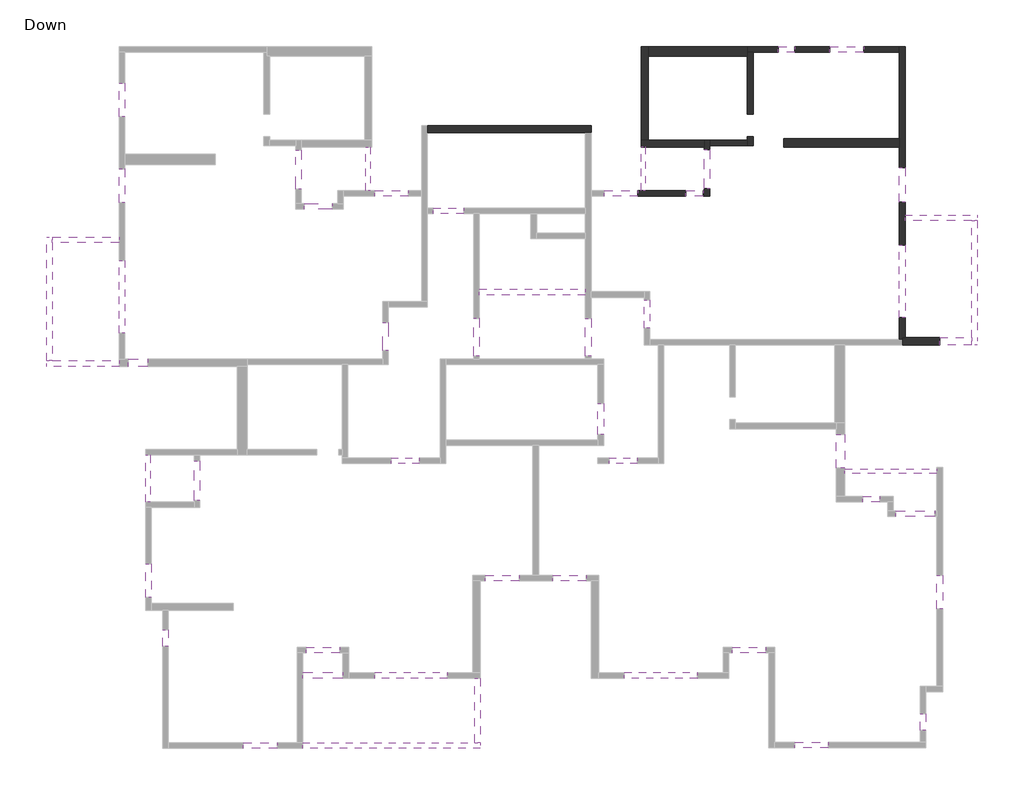
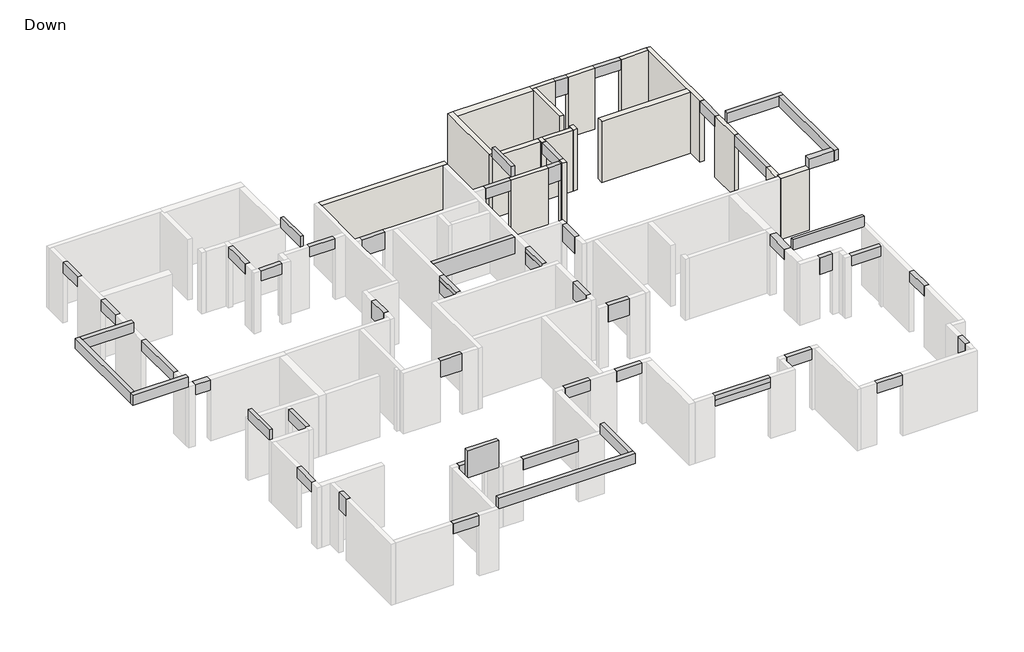
# One storey, part 3 of 3: 52 beams, 19 walls.
"""IFC4 building model written with IfcOpenShell, lengths in millimetres."""

from ifc_helpers import new_model, si_unit, frame, origin, place, context, project, spatial, polyline, outline, extrude, faceted_brep, element, save

model = new_model("IFC4")

# Units and contexts
model_context = context("Model", 3, world=origin())
ifc_project = project(units=[si_unit("LENGTHUNIT", "METRE", prefix="MILLI")], contexts=[model_context])

# Site, building, storey
site = spatial("IfcSite", under=ifc_project)
building = spatial("IfcBuilding", under=site)
storey = spatial("IfcBuildingStorey", under=building, Name="Down", Elevation=0.0)

# Beams
placement = place(None, origin())
element("IfcBeam", 1, ObjectType="Concrete Rectengular Beam : 15/50", at=placement, inside=storey, context=model_context, shape_type="SweptSolid", body=[
    extrude(outline(polyline([(18937.905294, -3693.5538503), (18937.905294, -3843.5538503), (15639.9526685, -3843.5538503), (15639.9526685, -3693.5538503), (18937.905294, -3693.5538503)])), frame((0.0, 0.0, 3000.0), z_axis=(0.0, 0.0, 1.0), x_axis=(1.0, 0.0, 0.0)), (0.0, 0.0, 1.0), 500.0),
])
element("IfcBeam", 2, ObjectType="Concrete Rectengular Beam : 15/50", at=placement, inside=storey, context=model_context, shape_type="SweptSolid", body=[
    extrude(outline(polyline([(8357.905294, 7842.0164502), (8507.905294, 7842.0164502), (8507.905294, 6284.3445962), (8357.905294, 6284.3445962), (8357.905294, 7842.0164502)])), frame((0.0, 0.0, 3000.0), z_axis=(0.0, 0.0, 1.0), x_axis=(1.0, 0.0, 0.0)), (0.0, 0.0, 1.0), 500.0),
])
element("IfcBeam", 3, ObjectType="Concrete Rectengular Beam : 15/50", at=placement, inside=storey, context=model_context, shape_type="SweptSolid", body=[
    extrude(outline(polyline([(-1489.8370837, 7836.068874), (-1339.8370837, 7836.068874), (-1339.8370837, 6280.1520062), (-1489.8370837, 6280.1520062), (-1489.8370837, 7836.068874)])), frame((0.0, 0.0, 3000.0), z_axis=(0.0, 0.0, 1.0), x_axis=(1.0, 0.0, 0.0)), (0.0, 0.0, 1.0), 500.0),
])
element("IfcBeam", 4, ObjectType="Concrete Rectengular Beam : 15/50", at=placement, inside=storey, context=model_context, shape_type="SweptSolid", body=[
    extrude(outline(polyline([(-9364.7328942, -3194.7427075), (-9214.7328942, -3194.7427075), (-9214.7328942, -4872.9835498), (-9364.7328942, -4872.9835498), (-9364.7328942, -3194.7427075)])), frame((0.0, 0.0, 3000.0), z_axis=(0.0, 0.0, 1.0), x_axis=(1.0, 0.0, 0.0)), (0.0, 0.0, 1.0), 500.0),
])
element("IfcBeam", 5, ObjectType="Concrete Rectengular Beam : 20/133", at=placement, inside=storey, context=model_context, shape_type="SweptSolid", body=[
    extrude(outline(polyline([(-3754.594706, -11177.9835498), (-3754.594706, -10977.9835498), (-2314.594706, -10977.9835498), (-2314.594706, -11177.9835498), (-3754.594706, -11177.9835498)])), frame((0.0, 0.0, 3000.0), z_axis=(0.0, 0.0, 1.0), x_axis=(1.0, 0.0, 0.0)), (0.0, 0.0, 1.0), 1330.0),
])
element("IfcBeam", 6, ObjectType="Concrete Rectengular Beam : 20/50", at=placement, inside=storey, context=model_context, shape_type="Brep", body=[
    faceted_brep([(-3999.8370837, 7726.5624033, 3000.0), (-3799.8370837, 7726.5624033, 3000.0), (-3799.8370837, 7726.5624033, 2500.0), (-3999.8370837, 7726.5624033, 2500.0), (-3999.8370837, 7215.1187953, 3000.0), (-3999.8370837, 6335.1520062, 3000.0), (-3799.8370837, 6335.1520062, 3000.0), (-3799.8370837, 6335.1520062, 2500.0), (-3999.8370837, 6335.1520062, 2500.0)], [[[0, 1, 2, 3]], [[1, 0, 4, 5, 6]], [[2, 1, 6, 7]], [[3, 2, 7, 8]], [[0, 3, 8, 5, 4]], [[6, 5, 8, 7]]]),
])
element("IfcBeam", 7, ObjectType="Concrete Rectengular Beam : 20/50", at=placement, inside=storey, context=model_context, shape_type="SweptSolid", body=[
    extrude(outline(polyline([(-2696.679593, 5815.1520062), (-2696.679593, 5615.1520062), (-3696.679593, 5615.1520062), (-3696.679593, 5815.1520062), (-2696.679593, 5815.1520062)])), frame((0.0, 0.0, 2500.0), z_axis=(0.0, 0.0, 1.0), x_axis=(1.0, 0.0, 0.0)), (0.0, 0.0, 1.0), 500.0),
])
element("IfcBeam", 8, ObjectType="Concrete Rectengular Beam : 20/50", at=placement, inside=storey, context=model_context, shape_type="SweptSolid", body=[
    extrude(outline(polyline([(28.320407, 6280.1520062), (28.320407, 6080.1520062), (-1171.679593, 6080.1520062), (-1171.679593, 6280.1520062), (28.320407, 6280.1520062)])), frame((0.0, 0.0, 2500.0), z_axis=(0.0, 0.0, 1.0), x_axis=(1.0, 0.0, 0.0)), (0.0, 0.0, 1.0), 500.0),
])
element("IfcBeam", 9, ObjectType="Concrete Rectengular Beam : 20/50", at=placement, inside=storey, context=model_context, shape_type="SweptSolid", body=[
    extrude(outline(polyline([(-10319.6462524, 10130.5632806), (-10119.6462524, 10130.5632806), (-10119.6462524, 8930.3987709), (-10319.6462524, 8930.3987709), (-10319.6462524, 10130.5632806)])), frame((0.0, 0.0, 2500.0), z_axis=(0.0, 0.0, 1.0), x_axis=(1.0, 0.0, 0.0)), (0.0, 0.0, 1.0), 500.0),
])
element("IfcBeam", 10, ObjectType="Concrete Rectengular Beam : 20/50", at=placement, inside=storey, context=model_context, shape_type="SweptSolid", body=[
    extrude(outline(polyline([(-10319.6462524, 7055.0094311), (-10119.6462524, 7055.0094311), (-10119.6462524, 5854.8449214), (-10319.6462524, 5854.8449214), (-10319.6462524, 7055.0094311)])), frame((0.0, 0.0, 2500.0), z_axis=(0.0, 0.0, 1.0), x_axis=(1.0, 0.0, 0.0)), (0.0, 0.0, 1.0), 500.0),
])
element("IfcBeam", 11, ObjectType="Concrete Rectengular Beam : 20/50", at=placement, inside=storey, context=model_context, shape_type="SweptSolid", body=[
    extrude(outline(polyline([(-10319.6462524, 3780.4865094), (-10119.6462524, 3780.4865094), (-10119.6462524, 1181.1884177), (-10319.6462524, 1181.1884177), (-10319.6462524, 3780.4865094)])), frame((0.0, 0.0, 2500.0), z_axis=(0.0, 0.0, 1.0), x_axis=(1.0, 0.0, 0.0)), (0.0, 0.0, 1.0), 500.0),
])
element("IfcBeam", 12, ObjectType="Concrete Rectengular Beam : 20/50", at=placement, inside=storey, context=model_context, shape_type="SweptSolid", body=[
    extrude(outline(polyline([(-7634.594706, -3392.9835498), (-7434.594706, -3392.9835498), (-7434.594706, -4812.9835498), (-7634.594706, -4812.9835498), (-7634.594706, -3392.9835498)])), frame((0.0, 0.0, 2500.0), z_axis=(0.0, 0.0, 1.0), x_axis=(1.0, 0.0, 0.0)), (0.0, 0.0, 1.0), 500.0),
])
element("IfcBeam", 13, ObjectType="Concrete Rectengular Beam : 20/50", at=placement, inside=storey, context=model_context, shape_type="SweptSolid", body=[
    extrude(outline(polyline([(-9364.594706, -7092.9835498), (-9164.594706, -7092.9835498), (-9164.594706, -8292.9835498), (-9364.594706, -8292.9835498), (-9364.594706, -7092.9835498)])), frame((0.0, 0.0, 2500.0), z_axis=(0.0, 0.0, 1.0), x_axis=(1.0, 0.0, 0.0)), (0.0, 0.0, 1.0), 500.0),
])
element("IfcBeam", 14, ObjectType="Concrete Rectengular Beam : 20/50", at=placement, inside=storey, context=model_context, shape_type="SweptSolid", body=[
    extrude(outline(polyline([(-5884.594706, -13682.9835498), (-5884.594706, -13482.9835498), (-4664.594706, -13482.9835498), (-4664.594706, -13682.9835498), (-5884.594706, -13682.9835498)])), frame((0.0, 0.0, 2500.0), z_axis=(0.0, 0.0, 1.0), x_axis=(1.0, 0.0, 0.0)), (0.0, 0.0, 1.0), 500.0),
])
element("IfcBeam", 15, ObjectType="Concrete Rectengular Beam : 20/50", at=placement, inside=storey, context=model_context, shape_type="SweptSolid", body=[
    extrude(outline(polyline([(-3634.594706, -10272.9835498), (-3634.594706, -10072.9835498), (-2434.594706, -10072.9835498), (-2434.594706, -10272.9835498), (-3634.594706, -10272.9835498)])), frame((0.0, 0.0, 2500.0), z_axis=(0.0, 0.0, 1.0), x_axis=(1.0, 0.0, 0.0)), (0.0, 0.0, 1.0), 500.0),
])
element("IfcBeam", 16, ObjectType="Concrete Rectengular Beam : 20/50", at=placement, inside=storey, context=model_context, shape_type="SweptSolid", body=[
    extrude(outline(polyline([(-1184.594706, -11177.9835498), (-1184.594706, -10977.9835498), (1415.405294, -10977.9835498), (1415.405294, -11177.9835498), (-1184.594706, -11177.9835498)])), frame((0.0, 0.0, 2500.0), z_axis=(0.0, 0.0, 1.0), x_axis=(1.0, 0.0, 0.0)), (0.0, 0.0, 1.0), 500.0),
])
element("IfcBeam", 17, ObjectType="Concrete Rectengular Beam : 20/50", at=placement, inside=storey, context=model_context, shape_type="SweptSolid", body=[
    extrude(outline(polyline([(2785.405294, -7702.9835498), (2785.405294, -7502.9835498), (3985.405294, -7502.9835498), (3985.405294, -7702.9835498), (2785.405294, -7702.9835498)])), frame((0.0, 0.0, 2500.0), z_axis=(0.0, 0.0, 1.0), x_axis=(1.0, 0.0, 0.0)), (0.0, 0.0, 1.0), 500.0),
])
element("IfcBeam", 18, ObjectType="Concrete Rectengular Beam : 20/50", at=placement, inside=storey, context=model_context, shape_type="SweptSolid", body=[
    extrude(outline(polyline([(5185.405294, -7702.9835498), (5185.405294, -7502.9835498), (6385.405294, -7502.9835498), (6385.405294, -7702.9835498), (5185.405294, -7702.9835498)])), frame((0.0, 0.0, 2500.0), z_axis=(0.0, 0.0, 1.0), x_axis=(1.0, 0.0, 0.0)), (0.0, 0.0, 1.0), 500.0),
])
element("IfcBeam", 19, ObjectType="Concrete Rectengular Beam : 20/50", at=placement, inside=storey, context=model_context, shape_type="SweptSolid", body=[
    extrude(outline(polyline([(8239.9948169, 6284.3445962), (8239.9948169, 6084.3445962), (7043.320407, 6084.3445962), (7043.320407, 6284.3445962), (8239.9948169, 6284.3445962)])), frame((0.0, 0.0, 2500.0), z_axis=(0.0, 0.0, 1.0), x_axis=(1.0, 0.0, 0.0)), (0.0, 0.0, 1.0), 500.0),
])
element("IfcBeam", 20, ObjectType="Concrete Rectengular Beam : 20/50", at=placement, inside=storey, context=model_context, shape_type="Brep", body=[
    faceted_brep([(10617.905294, 7752.0164502, 3000.0), (10817.905294, 7752.0164502, 3000.0), (10817.905294, 7752.0164502, 2780.0), (10817.905294, 7752.0164502, 2500.0), (10617.905294, 7752.0164502, 2500.0), (10617.905294, 6354.3445962, 3000.0), (10817.905294, 6354.3445962, 3000.0), (10817.905294, 6354.3445962, 2500.0), (10617.905294, 6354.3445962, 2500.0)], [[[0, 1, 2, 3, 4]], [[1, 0, 5, 6]], [[2, 1, 6, 7, 3]], [[4, 3, 7, 8]], [[0, 4, 8, 5]], [[6, 5, 8, 7]]]),
])
element("IfcBeam", 21, ObjectType="Concrete Rectengular Beam : 20/50", at=placement, inside=storey, context=model_context, shape_type="SweptSolid", body=[
    extrude(outline(polyline([(16317.905294, 11432.0164502), (16317.905294, 11232.0164502), (15097.905294, 11232.0164502), (15097.905294, 11432.0164502), (16317.905294, 11432.0164502)])), frame((0.0, 0.0, 2500.0), z_axis=(0.0, 0.0, 1.0), x_axis=(1.0, 0.0, 0.0)), (0.0, 0.0, 1.0), 500.0),
])
element("IfcBeam", 22, ObjectType="Concrete Rectengular Beam : 20/50", at=placement, inside=storey, context=model_context, shape_type="SweptSolid", body=[
    extrude(outline(polyline([(17797.905294, 5872.0164502), (17597.905294, 5872.0164502), (17597.905294, 7092.0164502), (17797.905294, 7092.0164502), (17797.905294, 5872.0164502)])), frame((0.0, 0.0, 2500.0), z_axis=(0.0, 0.0, 1.0), x_axis=(1.0, 0.0, 0.0)), (0.0, 0.0, 1.0), 500.0),
])
element("IfcBeam", 23, ObjectType="Concrete Rectengular Beam : 20/50", at=placement, inside=storey, context=model_context, shape_type="SweptSolid", body=[
    extrude(outline(polyline([(17797.905294, 1732.0164502), (17597.905294, 1732.0164502), (17597.905294, 4332.0164502), (17797.905294, 4332.0164502), (17797.905294, 1732.0164502)])), frame((0.0, 0.0, 2500.0), z_axis=(0.0, 0.0, 1.0), x_axis=(1.0, 0.0, 0.0)), (0.0, 0.0, 1.0), 500.0),
])
element("IfcBeam", 24, ObjectType="Concrete Rectengular Beam : 20/50", at=placement, inside=storey, context=model_context, shape_type="SweptSolid", body=[
    extrude(outline(polyline([(18857.905294, -5182.9835498), (18857.905294, -5382.9835498), (17457.905294, -5382.9835498), (17457.905294, -5182.9835498), (18857.905294, -5182.9835498)])), frame((0.0, 0.0, 2500.0), z_axis=(0.0, 0.0, 1.0), x_axis=(1.0, 0.0, 0.0)), (0.0, 0.0, 1.0), 500.0),
])
element("IfcBeam", 25, ObjectType="Concrete Rectengular Beam : 20/50", at=placement, inside=storey, context=model_context, shape_type="SweptSolid", body=[
    extrude(outline(polyline([(19137.905294, -8697.9835498), (18937.905294, -8697.9835498), (18937.905294, -7497.9835498), (19137.905294, -7497.9835498), (19137.905294, -8697.9835498)])), frame((0.0, 0.0, 2500.0), z_axis=(0.0, 0.0, 1.0), x_axis=(1.0, 0.0, 0.0)), (0.0, 0.0, 1.0), 500.0),
])
element("IfcBeam", 26, ObjectType="Concrete Rectengular Beam : 20/50", at=placement, inside=storey, context=model_context, shape_type="SweptSolid", body=[
    extrude(outline(polyline([(13857.905294, -13677.9835498), (13857.905294, -13477.9835498), (15057.905294, -13477.9835498), (15057.905294, -13677.9835498), (13857.905294, -13677.9835498)])), frame((0.0, 0.0, 2500.0), z_axis=(0.0, 0.0, 1.0), x_axis=(1.0, 0.0, 0.0)), (0.0, 0.0, 1.0), 500.0),
])
element("IfcBeam", 27, ObjectType="Concrete Rectengular Beam : 20/50", at=placement, inside=storey, context=model_context, shape_type="SweptSolid", body=[
    extrude(outline(polyline([(11607.905294, -10277.9835498), (11607.905294, -10077.9835498), (12807.905294, -10077.9835498), (12807.905294, -10277.9835498), (11607.905294, -10277.9835498)])), frame((0.0, 0.0, 2500.0), z_axis=(0.0, 0.0, 1.0), x_axis=(1.0, 0.0, 0.0)), (0.0, 0.0, 1.0), 500.0),
])
element("IfcBeam", 28, ObjectType="Concrete Rectengular Beam : 20/50", at=placement, inside=storey, context=model_context, shape_type="SweptSolid", body=[
    extrude(outline(polyline([(-11172.9835498, 3000.0), (-10977.9835498, 3000.0), (-10977.9835498, 2500.0), (-11177.9835498, 2500.0), (-11177.9835498, 2780.0), (-11172.9835498, 2780.0), (-11172.9835498, 3000.0)])), frame((7755.405294, 0.0, 0.0), z_axis=(1.0, 0.0, 0.0), x_axis=(0.0, 1.0, 0.0)), (0.0, 0.0, 1.0), 2602.5),
])
element("IfcBeam", 29, ObjectType="Concrete Rectengular Beam : 20/50", at=placement, inside=storey, context=model_context, shape_type="Brep", body=[
    faceted_brep([(-3754.594706, -13482.9835498, 3500.0), (-3754.594706, -13482.9835498, 3000.0), (-3754.594706, -13682.9835498, 3000.0), (-3754.594706, -13682.9835498, 3500.0), (2605.405294, -13682.9835498, 3500.0), (2605.405294, -13482.9835498, 3500.0), (2405.405294, -13482.9835498, 3500.0), (2605.405294, -13682.9835498, 3000.0), (2405.405294, -13482.9835498, 3000.0), (2605.405294, -13482.9835498, 3000.0)], [[[0, 1, 2, 3]], [[0, 3, 4, 5, 6]], [[3, 2, 7, 4]], [[2, 1, 8, 9, 7]], [[1, 0, 6, 5, 9, 8]], [[5, 4, 7, 9]]]),
])
element("IfcBeam", 30, ObjectType="Concrete Rectengular Beam : 20/50", at=placement, inside=storey, context=model_context, shape_type="SweptSolid", body=[
    extrude(outline(polyline([(2405.405294, -11177.9835498), (2605.405294, -11177.9835498), (2605.405294, -13482.9835498), (2405.405294, -13482.9835498), (2405.405294, -11177.9835498)])), frame((0.0, 0.0, 3000.0), z_axis=(0.0, 0.0, 1.0), x_axis=(1.0, 0.0, 0.0)), (0.0, 0.0, 1.0), 500.0),
])
element("IfcBeam", 31, ObjectType="Concrete Rectengular Beam : 20/50", at=placement, inside=storey, context=model_context, shape_type="Brep", body=[
    faceted_brep([(-10319.6462524, -12.6260152, 3500.0), (-10319.6462524, -12.6260152, 3000.0), (-10319.6462524, 187.3739848, 3000.0), (-10319.6462524, 187.3739848, 3500.0), (-12719.6462524, 187.3739848, 3500.0), (-12919.6462524, 187.3739848, 3500.0), (-12919.6462524, -12.6260152, 3500.0), (-12719.6462524, 187.3739848, 3000.0), (-12919.6462524, 187.3739848, 3000.0), (-12919.6462524, -12.6260152, 3000.0)], [[[0, 1, 2, 3]], [[0, 3, 4, 5, 6]], [[3, 2, 7, 8, 5, 4]], [[2, 1, 9, 8, 7]], [[1, 0, 6, 9]], [[6, 5, 8, 9]]]),
])
element("IfcBeam", 32, ObjectType="Concrete Rectengular Beam : 20/50", at=placement, inside=storey, context=model_context, shape_type="Brep", body=[
    faceted_brep([(-12719.6462524, 4616.1884177, 3500.0), (-12919.6462524, 4616.1884177, 3500.0), (-12919.6462524, 187.3739848, 3500.0), (-12719.6462524, 187.3739848, 3500.0), (-12719.6462524, 4416.1884177, 3500.0), (-12719.6462524, 4616.1884177, 3000.0), (-12719.6462524, 187.3739848, 3000.0), (-12719.6462524, 4416.1884177, 3000.0), (-12919.6462524, 4616.1884177, 3000.0), (-12919.6462524, 187.3739848, 3000.0)], [[[0, 1, 2, 3, 4]], [[5, 0, 4, 3, 6, 7]], [[8, 5, 7, 6, 9]], [[1, 8, 9, 2]], [[3, 2, 9, 6]], [[1, 0, 5, 8]]]),
])
element("IfcBeam", 33, ObjectType="Concrete Rectengular Beam : 20/50", at=placement, inside=storey, context=model_context, shape_type="SweptSolid", body=[
    extrude(outline(polyline([(-10319.6462524, 4616.1884177), (-10319.6462524, 4416.1884177), (-12719.6462524, 4416.1884177), (-12719.6462524, 4616.1884177), (-10319.6462524, 4616.1884177)])), frame((0.0, 0.0, 3000.0), z_axis=(0.0, 0.0, 1.0), x_axis=(1.0, 0.0, 0.0)), (0.0, 0.0, 1.0), 500.0),
])
element("IfcBeam", 34, ObjectType="Concrete Rectengular Beam : 20/50", at=placement, inside=storey, context=model_context, shape_type="Brep", body=[
    faceted_brep([(17797.905294, 5405.0203984, 3500.0), (17797.905294, 5405.0203984, 3000.0), (17797.905294, 5205.0203984, 3000.0), (17797.905294, 5205.0203984, 3500.0), (20188.2392489, 5205.0203984, 3500.0), (20388.2392489, 5205.0203984, 3500.0), (20388.2392489, 5405.0203984, 3500.0), (20188.2392489, 5205.0203984, 3000.0), (20388.2392489, 5205.0203984, 3000.0), (20388.2392489, 5405.0203984, 3000.0)], [[[0, 1, 2, 3]], [[0, 3, 4, 5, 6]], [[3, 2, 7, 8, 5, 4]], [[2, 1, 9, 8, 7]], [[1, 0, 6, 9]], [[6, 5, 8, 9]]]),
])
element("IfcBeam", 35, ObjectType="Concrete Rectengular Beam : 20/50", at=placement, inside=storey, context=model_context, shape_type="Brep", body=[
    faceted_brep([(20188.2392489, 752.0164502, 3500.0), (20388.2392489, 752.0164502, 3500.0), (20388.2392489, 5205.0203984, 3500.0), (20188.2392489, 5205.0203984, 3500.0), (20188.2392489, 1022.0164502, 3500.0), (20188.2392489, 752.0164502, 3000.0), (20188.2392489, 5205.0203984, 3000.0), (20188.2392489, 1022.0164502, 3000.0), (20388.2392489, 752.0164502, 3000.0), (20388.2392489, 5205.0203984, 3000.0), (20388.2392489, 1022.0164502, 3000.0)], [[[0, 1, 2, 3, 4]], [[5, 0, 4, 3, 6, 7]], [[8, 5, 7, 6, 9, 10]], [[1, 8, 10, 9, 2]], [[3, 2, 9, 6]], [[1, 0, 5, 8]]]),
])
element("IfcBeam", 36, ObjectType="Concrete Rectengular Beam : 20/82", at=placement, inside=storey, context=model_context, shape_type="SweptSolid", body=[
    extrude(outline(polyline([(-8764.594706, -9442.9835498), (-8564.594706, -9442.9835498), (-8564.594706, -10042.9835498), (-8764.594706, -10042.9835498), (-8764.594706, -9442.9835498)])), frame((0.0, 0.0, 2180.0), z_axis=(0.0, 0.0, 1.0), x_axis=(1.0, 0.0, 0.0)), (0.0, 0.0, 1.0), 820.0),
])
element("IfcBeam", 37, ObjectType="Concrete Rectengular Beam : 20/82", at=placement, inside=storey, context=model_context, shape_type="SweptSolid", body=[
    extrude(outline(polyline([(-591.3286388, -3494.0144776), (-591.3286388, -3294.0144776), (410.820407, -3294.0144776), (410.820407, -3494.0144776), (-591.3286388, -3494.0144776)])), frame((0.0, 0.0, 2180.0), z_axis=(0.0, 0.0, 1.0), x_axis=(1.0, 0.0, 0.0)), (0.0, 0.0, 1.0), 820.0),
])
element("IfcBeam", 38, ObjectType="Concrete Rectengular Beam : 20/82", at=placement, inside=storey, context=model_context, shape_type="SweptSolid", body=[
    extrude(outline(polyline([(8213.320407, -3297.9835498), (8213.320407, -3497.9835498), (7210.820407, -3497.9835498), (7210.820407, -3297.9835498), (8213.320407, -3297.9835498)])), frame((0.0, 0.0, 2180.0), z_axis=(0.0, 0.0, 1.0), x_axis=(1.0, 0.0, 0.0)), (0.0, 0.0, 1.0), 820.0),
])
element("IfcBeam", 39, ObjectType="Concrete Rectengular Beam : 20/82", at=placement, inside=storey, context=model_context, shape_type="SweptSolid", body=[
    extrude(outline(polyline([(7010.820407, -2447.6464385), (6810.820407, -2447.6464385), (6810.820407, -1347.6464385), (7010.820407, -1347.6464385), (7010.820407, -2447.6464385)])), frame((0.0, 0.0, 2180.0), z_axis=(0.0, 0.0, 1.0), x_axis=(1.0, 0.0, 0.0)), (0.0, 0.0, 1.0), 820.0),
])
element("IfcBeam", 40, ObjectType="Concrete Rectengular Beam : 20/82", at=placement, inside=storey, context=model_context, shape_type="SweptSolid", body=[
    extrude(outline(polyline([(3000.0, 2560.820407), (3000.0, 2363.3932055), (2780.0, 2363.3932055), (2780.0, 2360.820407), (2180.0, 2360.820407), (2180.0, 2560.820407), (3000.0, 2560.820407)])), frame((0.0, 352.3535615, 0.0), z_axis=(0.0, 1.0, 0.0), x_axis=(0.0, 0.0, 1.0)), (0.0, 0.0, 1.0), 1353.5222876),
])
element("IfcBeam", 41, ObjectType="Concrete Rectengular Beam : 20/82", at=placement, inside=storey, context=model_context, shape_type="SweptSolid", body=[
    extrude(outline(polyline([(3000.0, 6563.320407), (3000.0, 6368.320407), (2780.0, 6368.320407), (2780.0, 6363.320407), (2180.0, 6363.320407), (2180.0, 6563.320407), (3000.0, 6563.320407)])), frame((0.0, 352.3535615, 0.0), z_axis=(0.0, 1.0, 0.0), x_axis=(0.0, 0.0, 1.0)), (0.0, 0.0, 1.0), 1352.7984447),
])
element("IfcBeam", 42, ObjectType="Concrete Rectengular Beam : 20/82", at=placement, inside=storey, context=model_context, shape_type="SweptSolid", body=[
    extrude(outline(polyline([(8463.320407, 2355.1520062), (8663.320407, 2355.1520062), (8663.320407, 1352.0164502), (8463.320407, 1352.0164502), (8463.320407, 2355.1520062)])), frame((0.0, 0.0, 2180.0), z_axis=(0.0, 0.0, 1.0), x_axis=(1.0, 0.0, 0.0)), (0.0, 0.0, 1.0), 820.0),
])
element("IfcBeam", 43, ObjectType="Concrete Rectengular Beam : 20/82", at=placement, inside=storey, context=model_context, shape_type="SweptSolid", body=[
    extrude(outline(polyline([(-690.8131749, 556.7642019), (-890.8131749, 556.7642019), (-890.8131749, 1555.8429472), (-690.8131749, 1555.8429472), (-690.8131749, 556.7642019)])), frame((0.0, 0.0, 2180.0), z_axis=(0.0, 0.0, 1.0), x_axis=(1.0, 0.0, 0.0)), (0.0, 0.0, 1.0), 820.0),
])
element("IfcBeam", 44, ObjectType="Concrete Rectengular Beam : 20/82", at=placement, inside=storey, context=model_context, shape_type="SweptSolid", body=[
    extrude(outline(polyline([(909.4061714, 5455.8758492), (909.4061714, 5655.8758492), (2013.320407, 5655.8758492), (2013.320407, 5455.8758492), (909.4061714, 5455.8758492)])), frame((0.0, 0.0, 2180.0), z_axis=(0.0, 0.0, 1.0), x_axis=(1.0, 0.0, 0.0)), (0.0, 0.0, 1.0), 820.0),
])
element("IfcBeam", 45, ObjectType="Concrete Rectengular Beam : 20/82", at=placement, inside=storey, context=model_context, shape_type="Brep", body=[
    faceted_brep([(6363.320407, 2545.8758492, 3000.0), (6363.320407, 2745.8758492, 3000.0), (2560.820407, 2745.8758492, 3000.0), (2560.820407, 2545.8758492, 3000.0), (6363.320407, 2545.8758492, 2180.0), (6363.320407, 2545.8758492, 2780.0), (2560.820407, 2545.8758492, 2780.0), (2560.820407, 2545.8758492, 2180.0), (6363.320407, 2745.8758492, 2180.0), (2560.820407, 2745.8758492, 2180.0)], [[[0, 1, 2, 3]], [[4, 5, 0, 3, 6, 7]], [[8, 4, 7, 9]], [[1, 8, 9, 2]], [[1, 0, 5, 4, 8]], [[3, 2, 9, 7, 6]]]),
])
element("IfcBeam", 46, ObjectType="Concrete Rectengular Beam : 20/82", at=placement, inside=storey, context=model_context, shape_type="SweptSolid", body=[
    extrude(outline(polyline([(10569.9948169, 6284.3445962), (10569.9948169, 6084.3445962), (9959.9948169, 6084.3445962), (9959.9948169, 6284.3445962), (10569.9948169, 6284.3445962)])), frame((0.0, 0.0, 2180.0), z_axis=(0.0, 0.0, 1.0), x_axis=(1.0, 0.0, 0.0)), (0.0, 0.0, 1.0), 820.0),
])
element("IfcBeam", 47, ObjectType="Concrete Rectengular Beam : 20/82", at=placement, inside=storey, context=model_context, shape_type="SweptSolid", body=[
    extrude(outline(polyline([(13857.905294, 11432.0164502), (13857.905294, 11232.0164502), (13257.905294, 11232.0164502), (13257.905294, 11432.0164502), (13857.905294, 11432.0164502)])), frame((0.0, 0.0, 2180.0), z_axis=(0.0, 0.0, 1.0), x_axis=(1.0, 0.0, 0.0)), (0.0, 0.0, 1.0), 820.0),
])
element("IfcBeam", 48, ObjectType="Concrete Rectengular Beam : 20/82", at=placement, inside=storey, context=model_context, shape_type="SweptSolid", body=[
    extrude(outline(polyline([(16897.905294, -4662.9835498), (16897.905294, -4862.9835498), (16277.905294, -4862.9835498), (16277.905294, -4662.9835498), (16897.905294, -4662.9835498)])), frame((0.0, 0.0, 2180.0), z_axis=(0.0, 0.0, 1.0), x_axis=(1.0, 0.0, 0.0)), (0.0, 0.0, 1.0), 820.0),
])
element("IfcBeam", 49, ObjectType="Concrete Rectengular Beam : 20/82", at=placement, inside=storey, context=model_context, shape_type="SweptSolid", body=[
    extrude(outline(polyline([(18537.905294, -13047.9835498), (18337.905294, -13047.9835498), (18337.905294, -12447.9835498), (18537.905294, -12447.9835498), (18537.905294, -13047.9835498)])), frame((0.0, 0.0, 2180.0), z_axis=(0.0, 0.0, 1.0), x_axis=(1.0, 0.0, 0.0)), (0.0, 0.0, 1.0), 820.0),
])
element("IfcBeam", 50, ObjectType="Concrete Rectengular Beam : 27/50", at=placement, inside=storey, context=model_context, shape_type="SweptSolid", body=[
    extrude(outline(polyline([(-9999.6462524, -18.8115823), (-9999.6462524, 251.1884177), (-9290.9338154, 251.1884177), (-9290.9338154, -18.8115823), (-9999.6462524, -18.8115823)])), frame((0.0, 0.0, 2500.0), z_axis=(0.0, 0.0, 1.0), x_axis=(1.0, 0.0, 0.0)), (0.0, 0.0, 1.0), 500.0),
])
element("IfcBeam", 51, ObjectType="Concrete Rectengular Beam : 27/50", at=placement, inside=storey, context=model_context, shape_type="SweptSolid", body=[
    extrude(outline(polyline([(19037.905294, 752.0164502), (19037.905294, 1022.0164502), (20188.2392489, 1022.0164502), (20188.2392489, 752.0164502), (19037.905294, 752.0164502)])), frame((0.0, 0.0, 3000.0), z_axis=(0.0, 0.0, 1.0), x_axis=(1.0, 0.0, 0.0)), (0.0, 0.0, 1.0), 500.0),
])
element("IfcBeam", 52, ObjectType="Concrete Rectengular Beam : 30/50", at=placement, inside=storey, context=model_context, shape_type="SweptSolid", body=[
    extrude(outline(polyline([(15639.9526685, -3647.9835498), (15339.9526685, -3647.9835498), (15339.9526685, -2447.9835498), (15639.9526685, -2447.9835498), (15639.9526685, -3647.9835498)])), frame((0.0, 0.0, 2500.0), z_axis=(0.0, 0.0, 1.0), x_axis=(1.0, 0.0, 0.0)), (0.0, 0.0, 1.0), 500.0),
])

# Walls
element("IfcWall", 53, ObjectType="20", at=placement, inside=storey, context=model_context, shape_type="Brep", body=[
    faceted_brep([(17797.905294, 1022.0164502, 0.0), (17797.905294, 1732.0164502, 0.0), (17797.905294, 1732.0164502, 2500.0), (17797.905294, 1732.0164502, 3000.0), (17797.905294, 1022.0164502, 3000.0), (17797.905294, 1022.0164502, 2780.0), (17597.905294, 952.0164502, 0.0), (17597.905294, 952.0164502, 2780.0), (17597.905294, 952.0164502, 3000.0), (17597.905294, 1732.0164502, 3000.0), (17597.905294, 1732.0164502, 2500.0), (17597.905294, 1732.0164502, 0.0), (17697.905294, 1022.0164502, 0.0), (17697.905294, 952.0164502, 0.0), (17697.905294, 952.0164502, 3000.0), (17697.905294, 1022.0164502, 3000.0)], [[[0, 1, 2, 3, 4, 5]], [[6, 7, 8, 9, 10, 11]], [[1, 0, 12, 13, 6, 11]], [[3, 2, 1, 11, 10, 9]], [[4, 3, 9, 8, 14, 15]], [[0, 5, 4, 15, 12]], [[15, 14, 13, 12]], [[14, 8, 7, 6, 13]]]),
])
element("IfcWall", 54, ObjectType="20", at=placement, inside=storey, context=model_context, shape_type="Brep", body=[
    faceted_brep([(17797.905294, 4332.0164502, 0.0), (17797.905294, 5872.0164502, 0.0), (17797.905294, 5872.0164502, 2500.0), (17797.905294, 5872.0164502, 3000.0), (17797.905294, 5405.0203984, 3000.0), (17797.905294, 4332.0164502, 3000.0), (17797.905294, 4332.0164502, 2500.0), (17597.905294, 4332.0164502, 0.0), (17597.905294, 4332.0164502, 2500.0), (17597.905294, 4332.0164502, 3000.0), (17597.905294, 5872.0164502, 3000.0), (17597.905294, 5872.0164502, 2500.0), (17597.905294, 5872.0164502, 0.0)], [[[0, 1, 2, 3, 4, 5, 6]], [[7, 8, 9, 10, 11, 12]], [[1, 0, 7, 12]], [[3, 2, 1, 12, 11, 10]], [[5, 4, 3, 10, 9]], [[0, 6, 5, 9, 8, 7]]]),
])
element("IfcWall", 55, ObjectType="20", at=placement, inside=storey, context=model_context, shape_type="Brep", body=[
    faceted_brep([(17797.905294, 7092.0164502, 0.0), (17797.905294, 11432.0164502, 0.0), (17797.905294, 11432.0164502, 3000.0), (17797.905294, 7092.0164502, 3000.0), (17797.905294, 7092.0164502, 2500.0), (17597.905294, 7092.0164502, 0.0), (17597.905294, 7092.0164502, 2500.0), (17597.905294, 7092.0164502, 3000.0), (17597.905294, 7832.0164502, 3000.0), (17597.905294, 8132.0164502, 3000.0), (17597.905294, 11232.0164502, 3000.0), (17597.905294, 11432.0164502, 3000.0), (17597.905294, 11432.0164502, 0.0), (17597.905294, 11232.0164502, 0.0), (17597.905294, 8132.0164502, 0.0), (17597.905294, 7832.0164502, 0.0)], [[[0, 1, 2, 3, 4]], [[5, 6, 7, 8, 9, 10, 11, 12, 13, 14, 15]], [[1, 0, 5, 15, 14, 13, 12]], [[3, 2, 11, 10, 9, 8, 7]], [[0, 4, 3, 7, 6, 5]], [[2, 1, 12, 11]]]),
])
element("IfcWall", 56, ObjectType="20", at=placement, inside=storey, context=model_context, shape_type="Brep", body=[
    faceted_brep([(17597.905294, 11432.0164502, 0.0), (16317.905294, 11432.0164502, 0.0), (16317.905294, 11432.0164502, 2500.0), (16317.905294, 11432.0164502, 3000.0), (17597.905294, 11432.0164502, 3000.0), (17597.905294, 11232.0164502, 0.0), (17597.905294, 11232.0164502, 2780.0), (17597.905294, 11232.0164502, 3000.0), (16317.905294, 11232.0164502, 3000.0), (16317.905294, 11232.0164502, 2500.0), (16317.905294, 11232.0164502, 0.0)], [[[0, 1, 2, 3, 4]], [[5, 6, 7, 8, 9, 10]], [[1, 0, 5, 10]], [[3, 2, 1, 10, 9, 8]], [[4, 3, 8, 7]], [[0, 4, 7, 6, 5]]]),
])
element("IfcWall", 57, ObjectType="20", at=placement, inside=storey, context=model_context, shape_type="Brep", body=[
    faceted_brep([(15097.905294, 11432.0164502, 0.0), (13857.905294, 11432.0164502, 0.0), (13857.905294, 11432.0164502, 2180.0), (13857.905294, 11432.0164502, 3000.0), (15097.905294, 11432.0164502, 3000.0), (15097.905294, 11432.0164502, 2500.0), (15097.905294, 11232.0164502, 0.0), (15097.905294, 11232.0164502, 2500.0), (15097.905294, 11232.0164502, 3000.0), (13857.905294, 11232.0164502, 3000.0), (13857.905294, 11232.0164502, 2180.0), (13857.905294, 11232.0164502, 0.0)], [[[0, 1, 2, 3, 4, 5]], [[6, 7, 8, 9, 10, 11]], [[1, 0, 6, 11]], [[3, 2, 1, 11, 10, 9]], [[4, 3, 9, 8]], [[0, 5, 4, 8, 7, 6]]]),
])
element("IfcWall", 58, ObjectType="20", at=placement, inside=storey, context=model_context, shape_type="Brep", body=[
    faceted_brep([(13257.905294, 11432.0164502, 0.0), (12157.905294, 11432.0164502, 0.0), (12157.905294, 11432.0164502, 3000.0), (13257.905294, 11432.0164502, 3000.0), (13257.905294, 11432.0164502, 2180.0), (13257.905294, 11232.0164502, 0.0), (13257.905294, 11232.0164502, 2180.0), (13257.905294, 11232.0164502, 3000.0), (12357.905294, 11232.0164502, 3000.0), (12157.905294, 11232.0164502, 3000.0), (12157.905294, 11232.0164502, 0.0), (12357.905294, 11232.0164502, 0.0)], [[[0, 1, 2, 3, 4]], [[5, 6, 7, 8, 9, 10, 11]], [[1, 0, 5, 11, 10]], [[3, 2, 9, 8, 7]], [[0, 4, 3, 7, 6, 5]], [[2, 1, 10, 9]]]),
])
element("IfcWall", 59, ObjectType="20", at=placement, inside=storey, context=model_context, shape_type="Brep", body=[
    faceted_brep([(12157.905294, 11232.0164502, 0.0), (12157.905294, 11082.0164502, 0.0), (12157.905294, 9012.0164502, 0.0), (12157.905294, 9012.0164502, 2780.0), (12157.905294, 9012.0164502, 3000.0), (12157.905294, 11082.0164502, 3000.0), (12157.905294, 11232.0164502, 3000.0), (12357.905294, 11232.0164502, 0.0), (12357.905294, 11232.0164502, 2780.0), (12357.905294, 11232.0164502, 3000.0), (12357.905294, 9012.0164502, 3000.0), (12357.905294, 9012.0164502, 2780.0), (12357.905294, 9012.0164502, 0.0), (12162.905294, 9012.0164502, 3000.0)], [[[0, 1, 2, 3, 4, 5, 6]], [[7, 8, 9, 10, 11, 12]], [[2, 1, 0, 7, 12]], [[4, 3, 2, 12, 11, 10, 13]], [[6, 5, 4, 13, 10, 9]], [[0, 6, 9, 8, 7]]]),
])
element("IfcWall", 60, ObjectType="20", at=placement, inside=storey, context=model_context, shape_type="Brep", body=[
    faceted_brep([(12157.905294, 8212.0164502, 0.0), (12157.905294, 8092.0164502, 0.0), (12157.905294, 7892.0164502, 0.0), (12157.905294, 7892.0164502, 3000.0), (12157.905294, 8092.0164502, 3000.0), (12157.905294, 8212.0164502, 3000.0), (12157.905294, 8212.0164502, 2780.0), (12357.905294, 8212.0164502, 0.0), (12357.905294, 8212.0164502, 2780.0), (12357.905294, 8212.0164502, 3000.0), (12357.905294, 7892.0164502, 3000.0), (12357.905294, 7892.0164502, 2780.0), (12357.905294, 7892.0164502, 0.0), (12162.905294, 8212.0164502, 3000.0)], [[[0, 1, 2, 3, 4, 5, 6]], [[7, 8, 9, 10, 11, 12]], [[2, 1, 0, 7, 12]], [[5, 4, 3, 10, 9, 13]], [[0, 6, 5, 13, 9, 8, 7]], [[3, 2, 12, 11, 10]]]),
])
element("IfcWall", 61, ObjectType="20", at=placement, inside=storey, context=model_context, shape_type="Brep", body=[
    faceted_brep([(12157.905294, 8092.0164502, 0.0), (10817.905294, 8092.0164502, 0.0), (10817.905294, 8092.0164502, 3000.0), (12157.905294, 8092.0164502, 3000.0), (12157.905294, 8092.0164502, 2780.0), (12157.905294, 7892.0164502, 0.0), (12157.905294, 7892.0164502, 3000.0), (10817.905294, 7892.0164502, 3000.0), (10817.905294, 7892.0164502, 2780.0), (10817.905294, 7892.0164502, 0.0)], [[[0, 1, 2, 3, 4]], [[5, 6, 7, 8, 9]], [[1, 0, 5, 9]], [[3, 2, 7, 6]], [[0, 4, 3, 6, 5]], [[2, 1, 9, 8, 7]]]),
])
element("IfcWall", 62, ObjectType="20", at=placement, inside=storey, context=model_context, shape_type="Brep", body=[
    faceted_brep([(10617.905294, 8092.0164502, 0.0), (10617.905294, 7842.0164502, 0.0), (10617.905294, 7752.0164502, 0.0), (10617.905294, 7752.0164502, 2500.0), (10617.905294, 7752.0164502, 3000.0), (10617.905294, 7842.0164502, 3000.0), (10617.905294, 8092.0164502, 3000.0), (10817.905294, 8092.0164502, 0.0), (10817.905294, 8092.0164502, 3000.0), (10817.905294, 7892.0164502, 3000.0), (10817.905294, 7752.0164502, 3000.0), (10817.905294, 7752.0164502, 2500.0), (10817.905294, 7752.0164502, 0.0), (10817.905294, 7892.0164502, 0.0)], [[[0, 1, 2, 3, 4, 5, 6]], [[7, 8, 9, 10, 11, 12, 13]], [[2, 1, 0, 7, 13, 12]], [[4, 3, 2, 12, 11, 10]], [[6, 5, 4, 10, 9, 8]], [[0, 6, 8, 7]]]),
])
element("IfcWall", 63, ObjectType="20", at=placement, inside=storey, context=model_context, shape_type="Brep", body=[
    faceted_brep([(10617.905294, 6354.3445962, 0.0), (10617.905294, 6284.3445962, 0.0), (10617.905294, 6084.3445962, 0.0), (10617.905294, 6084.3445962, 3000.0), (10617.905294, 6284.3445962, 3000.0), (10617.905294, 6354.3445962, 3000.0), (10617.905294, 6354.3445962, 2500.0), (10817.905294, 6354.3445962, 0.0), (10817.905294, 6354.3445962, 2500.0), (10817.905294, 6354.3445962, 3000.0), (10817.905294, 6084.3445962, 3000.0), (10817.905294, 6084.3445962, 2780.0), (10817.905294, 6084.3445962, 0.0)], [[[0, 1, 2, 3, 4, 5, 6]], [[7, 8, 9, 10, 11, 12]], [[2, 1, 0, 7, 12]], [[5, 4, 3, 10, 9]], [[0, 6, 5, 9, 8, 7]], [[3, 2, 12, 11, 10]]]),
])
element("IfcWall", 64, ObjectType="20", at=placement, inside=storey, context=model_context, shape_type="Brep", body=[
    faceted_brep([(10617.905294, 6284.3445962, 0.0), (10569.9948169, 6284.3445962, 0.0), (10569.9948169, 6284.3445962, 2180.0), (10569.9948169, 6284.3445962, 3000.0), (10617.905294, 6284.3445962, 3000.0), (10617.905294, 6284.3445962, 2780.0), (10617.905294, 6084.3445962, 0.0), (10617.905294, 6084.3445962, 3000.0), (10569.9948169, 6084.3445962, 3000.0), (10569.9948169, 6084.3445962, 2180.0), (10569.9948169, 6084.3445962, 0.0)], [[[0, 1, 2, 3, 4, 5]], [[6, 7, 8, 9, 10]], [[1, 0, 6, 10]], [[3, 2, 1, 10, 9, 8]], [[4, 3, 8, 7]], [[0, 5, 4, 7, 6]]]),
])
element("IfcWall", 65, ObjectType="20", at=placement, inside=storey, context=model_context, shape_type="Brep", body=[
    faceted_brep([(9959.9948169, 6284.3445962, 0.0), (8239.9948169, 6284.3445962, 0.0), (8239.9948169, 6284.3445962, 2500.0), (8239.9948169, 6284.3445962, 3000.0), (8357.905294, 6284.3445962, 3000.0), (9959.9948169, 6284.3445962, 3000.0), (9959.9948169, 6284.3445962, 2180.0), (9959.9948169, 6084.3445962, 0.0), (9959.9948169, 6084.3445962, 2180.0), (9959.9948169, 6084.3445962, 3000.0), (8239.9948169, 6084.3445962, 3000.0), (8239.9948169, 6084.3445962, 2500.0), (8239.9948169, 6084.3445962, 0.0)], [[[0, 1, 2, 3, 4, 5, 6]], [[7, 8, 9, 10, 11, 12]], [[1, 0, 7, 12]], [[3, 2, 1, 12, 11, 10]], [[5, 4, 3, 10, 9]], [[0, 6, 5, 9, 8, 7]]]),
])
element("IfcWall", 66, ObjectType="25", at=placement, inside=storey, context=model_context, shape_type="Brep", body=[
    faceted_brep([(708.320407, 8355.1520062, 0.0), (6363.320407, 8355.1520062, 0.0), (6563.320407, 8355.1520062, 0.0), (6563.320407, 8355.1520062, 3000.0), (6363.320407, 8355.1520062, 3000.0), (2460.820407, 8355.1520062, 3000.0), (708.320407, 8355.1520062, 3000.0), (708.320407, 8355.1520062, 2780.0), (708.320407, 8605.1520062, 0.0), (708.320407, 8605.1520062, 3000.0), (6563.320407, 8605.1520062, 3000.0), (6563.320407, 8605.1520062, 0.0)], [[[0, 1, 2, 3, 4, 5, 6, 7]], [[8, 9, 10, 11]], [[2, 1, 0, 8, 11]], [[6, 5, 4, 3, 10, 9]], [[0, 7, 6, 9, 8]], [[3, 2, 11, 10]]]),
])
element("IfcWall", 67, ObjectType="25", at=placement, inside=storey, context=model_context, shape_type="Brep", body=[
    faceted_brep([(10617.905294, 8092.0164502, 0.0), (8607.905294, 8092.0164502, 0.0), (8357.905294, 8092.0164502, 0.0), (8357.905294, 8092.0164502, 3000.0), (8607.905294, 8092.0164502, 3000.0), (10617.905294, 8092.0164502, 3000.0), (10617.905294, 7842.0164502, 0.0), (10617.905294, 7842.0164502, 2780.0), (10617.905294, 7842.0164502, 3000.0), (8357.905294, 7842.0164502, 3000.0), (8357.905294, 7842.0164502, 2780.0), (8357.905294, 7842.0164502, 0.0)], [[[0, 1, 2, 3, 4, 5]], [[6, 7, 8, 9, 10, 11]], [[2, 1, 0, 6, 11]], [[5, 4, 3, 9, 8]], [[0, 5, 8, 7, 6]], [[3, 2, 11, 10, 9]]]),
])
element("IfcWall", 68, ObjectType="25", at=placement, inside=storey, context=model_context, shape_type="Brep", body=[
    faceted_brep([(8607.905294, 8092.0164502, 0.0), (8607.905294, 11082.0164502, 0.0), (8607.905294, 11432.0164502, 0.0), (8607.905294, 11432.0164502, 3000.0), (8607.905294, 11082.0164502, 3000.0), (8607.905294, 8092.0164502, 3000.0), (8607.905294, 8092.0164502, 2780.0), (8357.905294, 8092.0164502, 0.0), (8357.905294, 8092.0164502, 3000.0), (8357.905294, 11432.0164502, 3000.0), (8357.905294, 11432.0164502, 0.0)], [[[0, 1, 2, 3, 4, 5, 6]], [[7, 8, 9, 10]], [[2, 1, 0, 7, 10]], [[5, 4, 3, 9, 8]], [[0, 6, 5, 8, 7]], [[3, 2, 10, 9]]]),
])
element("IfcWall", 69, ObjectType="27", at=placement, inside=storey, context=model_context, shape_type="Brep", body=[
    faceted_brep([(17697.905294, 752.0164502, 0.0), (19037.905294, 752.0164502, 0.0), (19037.905294, 752.0164502, 2780.0), (19037.905294, 752.0164502, 3000.0), (17697.905294, 752.0164502, 3000.0), (17697.905294, 1022.0164502, 0.0), (17697.905294, 1022.0164502, 3000.0), (17797.905294, 1022.0164502, 3000.0), (19037.905294, 1022.0164502, 3000.0), (19037.905294, 1022.0164502, 2780.0), (19037.905294, 1022.0164502, 0.0), (17797.905294, 1022.0164502, 0.0), (17697.905294, 952.0164502, 0.0), (17697.905294, 952.0164502, 3000.0)], [[[0, 1, 2, 3, 4]], [[5, 6, 7, 8, 9, 10, 11]], [[1, 0, 12, 5, 11, 10]], [[3, 2, 1, 10, 9, 8]], [[4, 3, 8, 7, 6, 13]], [[0, 4, 13, 6, 5, 12]]]),
])
element("IfcWall", 70, ObjectType="30", at=placement, inside=storey, context=model_context, shape_type="Brep", body=[
    faceted_brep([(17597.905294, 8132.0164502, 0.0), (13457.905294, 8132.0164502, 0.0), (13457.905294, 8132.0164502, 2780.0), (13457.905294, 8132.0164502, 3000.0), (17597.905294, 8132.0164502, 3000.0), (17597.905294, 8132.0164502, 2780.0), (17597.905294, 7832.0164502, 0.0), (17597.905294, 7832.0164502, 2780.0), (17597.905294, 7832.0164502, 3000.0), (13457.905294, 7832.0164502, 3000.0), (13457.905294, 7832.0164502, 2780.0), (13457.905294, 7832.0164502, 0.0), (13457.905294, 7892.0164502, 3000.0)], [[[0, 1, 2, 3, 4, 5]], [[6, 7, 8, 9, 10, 11]], [[1, 0, 6, 11]], [[3, 2, 1, 11, 10, 9, 12]], [[4, 3, 12, 9, 8]], [[0, 5, 4, 8, 7, 6]]]),
])
element("IfcWall", 71, ObjectType="35", at=placement, inside=storey, context=model_context, shape_type="Brep", body=[
    faceted_brep([(8607.905294, 11082.0164502, 0.0), (12157.905294, 11082.0164502, 0.0), (12157.905294, 11082.0164502, 2780.0), (12157.905294, 11082.0164502, 3000.0), (8607.905294, 11082.0164502, 3000.0), (8607.905294, 11082.0164502, 2780.0), (8607.905294, 11432.0164502, 0.0), (8607.905294, 11432.0164502, 3000.0), (12157.905294, 11432.0164502, 3000.0), (12157.905294, 11432.0164502, 0.0), (12157.905294, 11232.0164502, 0.0), (12157.905294, 11232.0164502, 3000.0)], [[[0, 1, 2, 3, 4, 5]], [[6, 7, 8, 9]], [[1, 0, 6, 9, 10]], [[4, 3, 11, 8, 7]], [[3, 2, 1, 10, 9, 8, 11]], [[0, 5, 4, 7, 6]]]),
])

save(model, "model.ifc")

# Revit data of these elements
# Type "Concrete Rectengular Beam : 15/50"
#   Length [instance default] = 152.4 cm
#   b = 15 cm
#   h = 50 cm
#   Structural Material [instance default] = Concrete
#   Assembly Code = ""
# Type "Concrete Rectengular Beam : 20/133"
#   Length [instance default] = 152.4 cm
#   b = 20 cm
#   h = 133 cm
#   Structural Material [instance default] = Concrete
#   Assembly Code = ""
# Type "Concrete Rectengular Beam : 20/50"
#   Length [instance default] = 152.4 cm
#   b = 20 cm
#   h = 50 cm
#   Structural Material [instance default] = Concrete
#   Assembly Code = ""
# Type "Concrete Rectengular Beam : 20/82"
#   Length [instance default] = 152.4 cm
#   b = 20 cm
#   h = 82 cm
#   Structural Material [instance default] = Concrete
#   Assembly Code = ""
# Type "Concrete Rectengular Beam : 27/50"
#   Length [instance default] = 152.4 cm
#   b = 27 cm
#   h = 50 cm
#   Structural Material [instance default] = Concrete
#   Assembly Code = ""
# Type "Concrete Rectengular Beam : 30/50"
#   Length [instance default] = 152.4 cm
#   b = 30 cm
#   h = 50 cm
#   Structural Material [instance default] = Concrete
#   Assembly Code = ""
# Type "20"
#   Layers, outside or top first: 20 cm "Concrete" (function 1)
# Type "25"
#   Layers, outside or top first: 25 cm "Concrete" (function 1)
# Type "27"
#   Layers, outside or top first: 27 cm "Concrete" (function 1)
# Type "30"
#   Layers, outside or top first: 30 cm "Concrete" (function 1)
# Type "35"
#   Layers, outside or top first: 35 cm "Concrete" (function 1)
# Element 1 (IfcBeam, "Concrete Rectengular Beam : 15/50")
#   Comments = ""
#   Mark = "B1"
#   SOFiSTiK_AMG_Comments = ""
#   SOFiSTiK_AMG_Scheduled = yes
#   SOFiSTiK_AMG_Adjusted = yes
#   Structural Material = Concrete
#   Phase Created = New Construction
#   Materials on its faces: "Concrete"
# Element 2 (IfcBeam, "Concrete Rectengular Beam : 15/50")
#   Comments = ""
#   Mark = "B2"
#   SOFiSTiK_AMG_Comments = ""
#   SOFiSTiK_AMG_Scheduled = yes
#   SOFiSTiK_AMG_Adjusted = yes
#   Structural Material = Concrete
#   Phase Created = New Construction
#   Materials on its faces: "Concrete"
# Element 3 (IfcBeam, "Concrete Rectengular Beam : 15/50")
#   Comments = ""
#   Mark = "B3"
#   SOFiSTiK_AMG_Comments = ""
#   SOFiSTiK_AMG_Scheduled = yes
#   SOFiSTiK_AMG_Adjusted = yes
#   Structural Material = Concrete
#   Phase Created = New Construction
#   Materials on its faces: "Concrete"
# Element 4 (IfcBeam, "Concrete Rectengular Beam : 15/50")
#   Comments = ""
#   Mark = "B4"
#   SOFiSTiK_AMG_Comments = ""
#   SOFiSTiK_AMG_Scheduled = yes
#   SOFiSTiK_AMG_Adjusted = yes
#   Structural Material = Concrete
#   Phase Created = New Construction
#   Materials on its faces: "Concrete"
# Element 5 (IfcBeam, "Concrete Rectengular Beam : 20/133")
#   Comments = ""
#   Mark = "B5"
#   SOFiSTiK_AMG_Comments = ""
#   SOFiSTiK_AMG_Scheduled = yes
#   SOFiSTiK_AMG_Adjusted = yes
#   Structural Material = Concrete
#   Phase Created = New Construction
#   Materials on its faces: "Concrete"
# Element 6 (IfcBeam, "Concrete Rectengular Beam : 20/50")
#   Comments = ""
#   Mark = "B7"
#   SOFiSTiK_AMG_Comments = ""
#   SOFiSTiK_AMG_Scheduled = yes
#   SOFiSTiK_AMG_Adjusted = yes
#   Structural Material = Concrete
#   Phase Created = New Construction
#   Materials on its faces: "Concrete"
# Element 7 (IfcBeam, "Concrete Rectengular Beam : 20/50")
#   Comments = ""
#   Mark = "B8"
#   SOFiSTiK_AMG_Comments = ""
#   SOFiSTiK_AMG_Scheduled = yes
#   SOFiSTiK_AMG_Adjusted = yes
#   Structural Material = Concrete
#   Phase Created = New Construction
#   Materials on its faces: "Concrete"
# Element 8 (IfcBeam, "Concrete Rectengular Beam : 20/50")
#   Comments = ""
#   Mark = "B9"
#   SOFiSTiK_AMG_Comments = ""
#   SOFiSTiK_AMG_Scheduled = yes
#   SOFiSTiK_AMG_Adjusted = yes
#   Structural Material = Concrete
#   Phase Created = New Construction
#   Materials on its faces: "Concrete"
# Element 9 (IfcBeam, "Concrete Rectengular Beam : 20/50")
#   Comments = ""
#   Mark = "B10"
#   SOFiSTiK_AMG_Comments = ""
#   SOFiSTiK_AMG_Scheduled = yes
#   SOFiSTiK_AMG_Adjusted = yes
#   Structural Material = Concrete
#   Phase Created = New Construction
#   Materials on its faces: "Concrete"
# Element 10 (IfcBeam, "Concrete Rectengular Beam : 20/50")
#   Comments = ""
#   Mark = "B11"
#   SOFiSTiK_AMG_Comments = ""
#   SOFiSTiK_AMG_Scheduled = yes
#   SOFiSTiK_AMG_Adjusted = yes
#   Structural Material = Concrete
#   Phase Created = New Construction
#   Materials on its faces: "Concrete"
# Element 11 (IfcBeam, "Concrete Rectengular Beam : 20/50")
#   Comments = ""
#   Mark = "B12"
#   SOFiSTiK_AMG_Comments = ""
#   SOFiSTiK_AMG_Scheduled = yes
#   SOFiSTiK_AMG_Adjusted = yes
#   Structural Material = Concrete
#   Phase Created = New Construction
#   Materials on its faces: "Concrete"
# Element 12 (IfcBeam, "Concrete Rectengular Beam : 20/50")
#   Comments = ""
#   Mark = "B13"
#   SOFiSTiK_AMG_Comments = ""
#   SOFiSTiK_AMG_Scheduled = yes
#   SOFiSTiK_AMG_Adjusted = yes
#   Structural Material = Concrete
#   Phase Created = New Construction
#   Materials on its faces: "Concrete"
# Element 13 (IfcBeam, "Concrete Rectengular Beam : 20/50")
#   Comments = ""
#   Mark = "B14"
#   SOFiSTiK_AMG_Comments = ""
#   SOFiSTiK_AMG_Scheduled = yes
#   SOFiSTiK_AMG_Adjusted = yes
#   Structural Material = Concrete
#   Phase Created = New Construction
#   Materials on its faces: "Concrete"
# Element 14 (IfcBeam, "Concrete Rectengular Beam : 20/50")
#   Comments = ""
#   Mark = "B15"
#   SOFiSTiK_AMG_Comments = ""
#   SOFiSTiK_AMG_Scheduled = yes
#   SOFiSTiK_AMG_Adjusted = yes
#   Structural Material = Concrete
#   Phase Created = New Construction
#   Materials on its faces: "Concrete"
# Element 15 (IfcBeam, "Concrete Rectengular Beam : 20/50")
#   Comments = ""
#   Mark = "B16"
#   SOFiSTiK_AMG_Comments = ""
#   SOFiSTiK_AMG_Scheduled = yes
#   SOFiSTiK_AMG_Adjusted = yes
#   Structural Material = Concrete
#   Phase Created = New Construction
#   Materials on its faces: "Concrete"
# Element 16 (IfcBeam, "Concrete Rectengular Beam : 20/50")
#   Comments = ""
#   Mark = "B17"
#   SOFiSTiK_AMG_Comments = ""
#   SOFiSTiK_AMG_Scheduled = yes
#   SOFiSTiK_AMG_Adjusted = yes
#   Structural Material = Concrete
#   Phase Created = New Construction
#   Materials on its faces: "Concrete"
# Element 17 (IfcBeam, "Concrete Rectengular Beam : 20/50")
#   Comments = ""
#   Mark = "B18"
#   SOFiSTiK_AMG_Comments = ""
#   SOFiSTiK_AMG_Scheduled = yes
#   SOFiSTiK_AMG_Adjusted = yes
#   Structural Material = Concrete
#   Phase Created = New Construction
#   Materials on its faces: "Concrete"
# Element 18 (IfcBeam, "Concrete Rectengular Beam : 20/50")
#   Comments = ""
#   Mark = "B19"
#   SOFiSTiK_AMG_Comments = ""
#   SOFiSTiK_AMG_Scheduled = yes
#   SOFiSTiK_AMG_Adjusted = yes
#   Structural Material = Concrete
#   Phase Created = New Construction
#   Materials on its faces: "Concrete"
# Element 19 (IfcBeam, "Concrete Rectengular Beam : 20/50")
#   Comments = ""
#   Mark = "B20"
#   SOFiSTiK_AMG_Comments = ""
#   SOFiSTiK_AMG_Scheduled = yes
#   SOFiSTiK_AMG_Adjusted = yes
#   Structural Material = Concrete
#   Phase Created = New Construction
#   Materials on its faces: "Concrete"
# Element 20 (IfcBeam, "Concrete Rectengular Beam : 20/50")
#   Comments = ""
#   Mark = "B21"
#   SOFiSTiK_AMG_Comments = ""
#   SOFiSTiK_AMG_Scheduled = yes
#   SOFiSTiK_AMG_Adjusted = yes
#   Structural Material = Concrete
#   Phase Created = New Construction
#   Materials on its faces: "Concrete"
# Element 21 (IfcBeam, "Concrete Rectengular Beam : 20/50")
#   Comments = ""
#   Mark = "B22"
#   SOFiSTiK_AMG_Comments = ""
#   SOFiSTiK_AMG_Scheduled = yes
#   SOFiSTiK_AMG_Adjusted = yes
#   Structural Material = Concrete
#   Phase Created = New Construction
#   Materials on its faces: "Concrete"
# Element 22 (IfcBeam, "Concrete Rectengular Beam : 20/50")
#   Comments = ""
#   Mark = "B23"
#   SOFiSTiK_AMG_Comments = ""
#   SOFiSTiK_AMG_Scheduled = yes
#   SOFiSTiK_AMG_Adjusted = yes
#   Structural Material = Concrete
#   Phase Created = New Construction
#   Materials on its faces: "Concrete"
# Element 23 (IfcBeam, "Concrete Rectengular Beam : 20/50")
#   Comments = ""
#   Mark = "B24"
#   SOFiSTiK_AMG_Comments = ""
#   SOFiSTiK_AMG_Scheduled = yes
#   SOFiSTiK_AMG_Adjusted = yes
#   Structural Material = Concrete
#   Phase Created = New Construction
#   Materials on its faces: "Concrete"
# Element 24 (IfcBeam, "Concrete Rectengular Beam : 20/50")
#   Comments = ""
#   Mark = "B25"
#   SOFiSTiK_AMG_Comments = ""
#   SOFiSTiK_AMG_Scheduled = yes
#   SOFiSTiK_AMG_Adjusted = yes
#   Structural Material = Concrete
#   Phase Created = New Construction
#   Materials on its faces: "Concrete"
# Element 25 (IfcBeam, "Concrete Rectengular Beam : 20/50")
#   Comments = ""
#   Mark = "B26"
#   SOFiSTiK_AMG_Comments = ""
#   SOFiSTiK_AMG_Scheduled = yes
#   SOFiSTiK_AMG_Adjusted = yes
#   Structural Material = Concrete
#   Phase Created = New Construction
#   Materials on its faces: "Concrete"
# Element 26 (IfcBeam, "Concrete Rectengular Beam : 20/50")
#   Comments = ""
#   Mark = "B27"
#   SOFiSTiK_AMG_Comments = ""
#   SOFiSTiK_AMG_Scheduled = yes
#   SOFiSTiK_AMG_Adjusted = yes
#   Structural Material = Concrete
#   Phase Created = New Construction
#   Materials on its faces: "Concrete"
# Element 27 (IfcBeam, "Concrete Rectengular Beam : 20/50")
#   Comments = ""
#   Mark = "B28"
#   SOFiSTiK_AMG_Comments = ""
#   SOFiSTiK_AMG_Scheduled = yes
#   SOFiSTiK_AMG_Adjusted = yes
#   Structural Material = Concrete
#   Phase Created = New Construction
#   Materials on its faces: "Concrete"
# Element 28 (IfcBeam, "Concrete Rectengular Beam : 20/50")
#   Comments = ""
#   Mark = "B29"
#   SOFiSTiK_AMG_Comments = ""
#   SOFiSTiK_AMG_Scheduled = yes
#   SOFiSTiK_AMG_Adjusted = yes
#   Structural Material = Concrete
#   Phase Created = New Construction
#   Materials on its faces: "Concrete"
# Element 29 (IfcBeam, "Concrete Rectengular Beam : 20/50")
#   Comments = ""
#   Mark = "B30"
#   SOFiSTiK_AMG_Comments = ""
#   SOFiSTiK_AMG_Scheduled = yes
#   SOFiSTiK_AMG_Adjusted = yes
#   Structural Material = Concrete
#   Phase Created = New Construction
#   Materials on its faces: "Concrete"
# Element 30 (IfcBeam, "Concrete Rectengular Beam : 20/50")
#   Comments = ""
#   Mark = "B31"
#   SOFiSTiK_AMG_Comments = ""
#   SOFiSTiK_AMG_Scheduled = yes
#   SOFiSTiK_AMG_Adjusted = yes
#   Structural Material = Concrete
#   Phase Created = New Construction
#   Materials on its faces: "Concrete"
# Element 31 (IfcBeam, "Concrete Rectengular Beam : 20/50")
#   Comments = ""
#   Mark = "B34"
#   SOFiSTiK_AMG_Comments = ""
#   SOFiSTiK_AMG_Scheduled = yes
#   SOFiSTiK_AMG_Adjusted = yes
#   Structural Material = Concrete
#   Phase Created = New Construction
#   Materials on its faces: "Concrete"
# Element 32 (IfcBeam, "Concrete Rectengular Beam : 20/50")
#   Comments = ""
#   Mark = "B35"
#   SOFiSTiK_AMG_Comments = ""
#   SOFiSTiK_AMG_Scheduled = yes
#   SOFiSTiK_AMG_Adjusted = yes
#   Structural Material = Concrete
#   Phase Created = New Construction
#   Materials on its faces: "Concrete"
# Element 33 (IfcBeam, "Concrete Rectengular Beam : 20/50")
#   Comments = ""
#   Mark = "B36"
#   SOFiSTiK_AMG_Comments = ""
#   SOFiSTiK_AMG_Scheduled = yes
#   SOFiSTiK_AMG_Adjusted = yes
#   Structural Material = Concrete
#   Phase Created = New Construction
#   Materials on its faces: "Concrete"
# Element 34 (IfcBeam, "Concrete Rectengular Beam : 20/50")
#   Comments = ""
#   Mark = "B37"
#   SOFiSTiK_AMG_Comments = ""
#   SOFiSTiK_AMG_Scheduled = yes
#   SOFiSTiK_AMG_Adjusted = yes
#   Structural Material = Concrete
#   Phase Created = New Construction
#   Materials on its faces: "Concrete"
# Element 35 (IfcBeam, "Concrete Rectengular Beam : 20/50")
#   Comments = ""
#   Mark = "B38"
#   SOFiSTiK_AMG_Comments = ""
#   SOFiSTiK_AMG_Scheduled = yes
#   SOFiSTiK_AMG_Adjusted = yes
#   Structural Material = Concrete
#   Phase Created = New Construction
#   Materials on its faces: "Concrete"
# Element 36 (IfcBeam, "Concrete Rectengular Beam : 20/82")
#   Comments = ""
#   Mark = "B39"
#   SOFiSTiK_AMG_Comments = ""
#   SOFiSTiK_AMG_Scheduled = yes
#   SOFiSTiK_AMG_Adjusted = yes
#   Structural Material = Concrete
#   Phase Created = New Construction
#   Materials on its faces: "Concrete"
# Element 37 (IfcBeam, "Concrete Rectengular Beam : 20/82")
#   Comments = ""
#   Mark = "B40"
#   SOFiSTiK_AMG_Comments = ""
#   SOFiSTiK_AMG_Scheduled = yes
#   SOFiSTiK_AMG_Adjusted = yes
#   Structural Material = Concrete
#   Phase Created = New Construction
#   Materials on its faces: "Concrete"
# Element 38 (IfcBeam, "Concrete Rectengular Beam : 20/82")
#   Comments = ""
#   Mark = "B41"
#   SOFiSTiK_AMG_Comments = ""
#   SOFiSTiK_AMG_Scheduled = yes
#   SOFiSTiK_AMG_Adjusted = yes
#   Structural Material = Concrete
